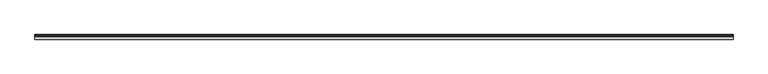
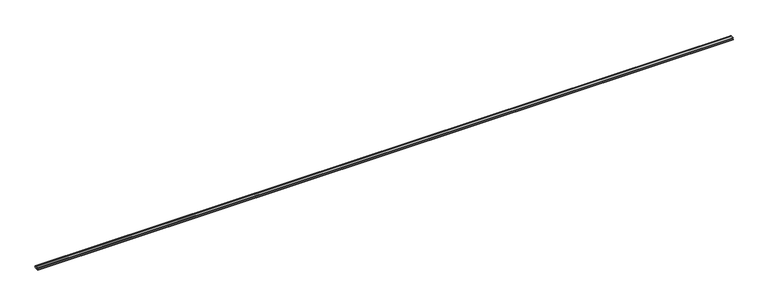
"""IFC4 building model written with IfcOpenShell, lengths in millimetres: proxy geometry, Generic Models 6:Generic Models 2:318829:Generic Models 2:318829 : Generic Models 6:Generic Models 2:318829:8 : Generic Models 6:Generic Models 2:318829:Generic Models 2:318829 : Generic Models 6:Generic Models 2:318829:300683."""

import ifcopenshell
import ifcopenshell.guid

model = None  # the IFC model being written
_history = None  # IfcOwnerHistory: only IFC2X3 demands one
_inside = {}  # id of a spatial element -> (the spatial element, [elements in it])
_under = {}  # id of a project, library or spatial element -> (it, [spatial elements below it])
_declared = {}  # id of a project -> (the project, [libraries it declares])
_typed = {}  # id of a type object -> (the type object, [elements of that type])
_made_of = {}  # id of a material, layer set ... -> (it, [elements and type objects made of it])


def new_model(schema):
    """Start an empty IFC model of exactly this schema.

    Asked for "IFC4X3", IfcOpenShell would pick the latest addendum, in which some entities
    have other attributes; the version numbers below select the first issue.
    IFC2X3 requires an IfcOwnerHistory on every rooted entity: one is made here for all.
    """
    global model, _history
    if schema == "IFC4X3":
        model = ifcopenshell.file(schema_version=(4, 3, 0, 0))
    else:
        model = ifcopenshell.file(schema=schema)
    _inside.clear()
    _under.clear()
    _declared.clear()
    _typed.clear()
    _made_of.clear()
    _history = None
    if model.schema == "IFC2X3":
        org = make("IfcOrganization", Name="unknown")
        user = make(
            "IfcPersonAndOrganization",
            ThePerson=make("IfcPerson", FamilyName="unknown"),
            TheOrganization=org,
        )
        app = make(
            "IfcApplication",
            ApplicationDeveloper=org,
            Version="unknown",
            ApplicationFullName="unknown",
            ApplicationIdentifier="unknown",
        )
        _history = make(
            "IfcOwnerHistory",
            OwningUser=user,
            OwningApplication=app,
            ChangeAction="ADDED",
            CreationDate=0,
        )
    return model


def make(cls, **values):
    """One entity of the class cls with the attributes given. An attribute that is None is left unset."""
    return model.create_entity(
        cls, **{name: value for name, value in values.items() if value is not None}
    )


def rooted(cls, **values):
    """An entity with a GlobalId (a new one), such as an element, a storey or a relation."""
    return make(cls, GlobalId=ifcopenshell.guid.new(), OwnerHistory=_history, **values)


def si_unit(unit_type, name, prefix=None):
    """IfcSIUnit, for example si_unit("LENGTHUNIT", "METRE", prefix="MILLI")."""
    return make("IfcSIUnit", UnitType=unit_type, Prefix=prefix, Name=name)


def assignment(units):
    """IfcUnitAssignment: the units of a project."""
    return None if units is None else make("IfcUnitAssignment", Units=units)


def point(xyz):
    """IfcCartesianPoint."""
    return None if xyz is None else make("IfcCartesianPoint", Coordinates=xyz)


def direction(xyz):
    """IfcDirection."""
    return None if xyz is None else make("IfcDirection", DirectionRatios=xyz)


def frame(location, z_axis=None, x_axis=None):
    """IfcAxis2Placement3D, a coordinate frame: its origin and axes. An axis left out is left unset."""
    return make(
        "IfcAxis2Placement3D",
        Location=point(location),
        Axis=direction(z_axis),
        RefDirection=direction(x_axis),
    )


def origin():
    """The frame at (0, 0, 0) with its axes left unset."""
    return frame((0.0, 0.0, 0.0))


def place(relative_to, where):
    """IfcLocalPlacement: puts the frame where relative to a parent placement (None: the world)."""
    return make(
        "IfcLocalPlacement", PlacementRelTo=relative_to, RelativePlacement=where
    )


def context(
    kind, dimensions, precision=None, world=None, true_north=None, identifier=None
):
    """IfcGeometricRepresentationContext, for example the 3D "Model" context."""
    return make(
        "IfcGeometricRepresentationContext",
        ContextIdentifier=identifier,
        ContextType=kind,
        CoordinateSpaceDimension=dimensions,
        Precision=precision,
        WorldCoordinateSystem=world,
        TrueNorth=true_north,
    )


def project(units=None, contexts=None):
    """IfcProject with its units and contexts."""
    return rooted(
        "IfcProject",
        Name="project",
        RepresentationContexts=contexts,
        UnitsInContext=assignment(units),
    )


def spatial(cls, under=None, at=None, **own):
    """A site, building, storey or space (cls), placed at a placement, below another one or the project."""
    s = rooted(cls, ObjectPlacement=at, **own)
    if under is not None:
        _under.setdefault(under.id(), (under, []))[1].append(s)
    return s


def polyline(points):
    """IfcPolyline through the points."""
    return make("IfcPolyline", Points=[point(p) for p in points])


def outline(outer, holes=None, kind="AREA"):
    """IfcArbitraryClosedProfileDef: a profile drawn as a closed curve; with holes, ...WithVoids."""
    if holes is None:
        return make("IfcArbitraryClosedProfileDef", ProfileType=kind, OuterCurve=outer)
    return make(
        "IfcArbitraryProfileDefWithVoids",
        ProfileType=kind,
        OuterCurve=outer,
        InnerCurves=holes,
    )


def extrude(swept, where, along, depth):
    """IfcExtrudedAreaSolid: the profile swept, set in the frame where, extruded along a direction by depth."""
    return make(
        "IfcExtrudedAreaSolid",
        SweptArea=swept,
        Position=where,
        ExtrudedDirection=direction(along),
        Depth=depth,
    )


def shape(context_of_items, identifier, shape_type, items):
    """IfcShapeRepresentation: the items that make up one representation, for example the "Body"."""
    return make(
        "IfcShapeRepresentation",
        ContextOfItems=context_of_items,
        RepresentationIdentifier=identifier,
        RepresentationType=shape_type,
        Items=items,
    )


def source(mapping_origin, context_of_items, identifier, shape_type, items):
    """IfcRepresentationMap: a shape defined once, which mapped items show again and again."""
    return make(
        "IfcRepresentationMap",
        MappingOrigin=mapping_origin,
        MappedRepresentation=shape(context_of_items, identifier, shape_type, items),
    )


def transform(
    local_origin,
    x_axis=None,
    y_axis=None,
    z_axis=None,
    scale=None,
    scale2=None,
    scale3=None,
    uniform=True,
):
    """IfcCartesianTransformationOperator3D, or its non-uniform kind. x_axis, y_axis, z_axis: its Axis1, 2, 3."""
    if uniform:
        return make(
            "IfcCartesianTransformationOperator3D",
            Axis1=direction(x_axis),
            Axis2=direction(y_axis),
            LocalOrigin=point(local_origin),
            Scale=scale,
            Axis3=direction(z_axis),
        )
    return make(
        "IfcCartesianTransformationOperator3DnonUniform",
        Axis1=direction(x_axis),
        Axis2=direction(y_axis),
        LocalOrigin=point(local_origin),
        Scale=scale,
        Axis3=direction(z_axis),
        Scale2=scale2,
        Scale3=scale3,
    )


def mapped(mapping_source, mapping_target):
    """IfcMappedItem: shows the shape of a source again, moved by a transform."""
    return make(
        "IfcMappedItem", MappingSource=mapping_source, MappingTarget=mapping_target
    )


def made_of(thing, what):
    """Note that an element or type object is made of a material, layer set ...; save() writes the relation."""
    if what is not None:
        _made_of.setdefault(what.id(), (what, []))[1].append(thing)
    return thing


def element(
    cls,
    number,
    at=None,
    inside=None,
    cuts=None,
    type_object=None,
    material=None,
    context=None,
    identifier="Body",
    shape_type=None,
    held_by="IfcProductDefinitionShape",
    body=None,
    shapes=None,
    **own,
):
    """One element of the class cls, such as IfcWall. Its Tag is "e" and its number.

    at: its placement. inside: the storey or other place that contains it. cuts: it is an
    opening in that element (IfcRelVoidsElement). A single representation is given by context,
    identifier, shape_type and body (its items); several are given by shapes. held_by: the class
    of the entity that holds the representations. save() writes the other relations.
    """
    e = rooted(cls, Tag="e%d" % number, ObjectPlacement=at, **own)
    if body is not None:
        shapes = [shape(context, identifier, shape_type, body)]
    if shapes is not None:
        e.Representation = make(held_by, Representations=shapes)
    if inside is not None:
        _inside.setdefault(inside.id(), (inside, []))[1].append(e)
    if cuts is not None:
        rooted(
            "IfcRelVoidsElement", RelatingBuildingElement=cuts, RelatedOpeningElement=e
        )
    if type_object is not None:
        _typed.setdefault(type_object.id(), (type_object, []))[1].append(e)
    return made_of(e, material)


def aggregate(whole, parts):
    """IfcRelAggregates: a whole, such as a stair, and the parts it consists of."""
    return rooted("IfcRelAggregates", RelatingObject=whole, RelatedObjects=parts)


def save(model, path):
    """Write the relations noted so far, then the file.

    IfcRelAggregates (storeys below a building ...), IfcRelContainedInSpatialStructure (elements
    in a storey), IfcRelDefinesByType, IfcRelAssociatesMaterial and IfcRelDeclares: one each for
    every whole, place, type object, material and project.
    """
    for whole, parts in _under.values():
        aggregate(whole, parts)
    for where, things in _inside.values():
        rooted(
            "IfcRelContainedInSpatialStructure",
            RelatedElements=things,
            RelatingStructure=where,
        )
    for kind, things in _typed.values():
        rooted("IfcRelDefinesByType", RelatedObjects=things, RelatingType=kind)
    for what, things in _made_of.values():
        rooted("IfcRelAssociatesMaterial", RelatedObjects=things, RelatingMaterial=what)
    for by, libraries in _declared.values():
        rooted("IfcRelDeclares", RelatingContext=by, RelatedDefinitions=libraries)
    model.write(path)


def generic_models_16859b6c(model_context):
    return source(origin(), model_context, "Body", "SweptSolid", [
        extrude(outline(polyline([(-579078.7997973, 0.0), (-579086.1349125, 0.0), (-579085.6631517, 1.207204), (-579085.2710441, 3.96875), (-579085.6631517, 6.730296), (-579086.1349125, 7.9375), (-579078.7997973, 7.9375), (-579080.7913182, 6.834014), (-579082.0090745, 5.2822838), (-579082.2625594, 3.5250635), (-579081.5121175, 1.8372538), (-579079.8751485, 0.482897), (-579078.7997973, 0.0)])), frame((590317.0242239, 0.0, 0.0), z_axis=(1.0, 0.0, 0.0), x_axis=(0.0, 1.0, 0.0)), (0.0, 0.0, 1.0), 2438.4),
        extrude(outline(polyline([(-579074.5205679, 0.0995049), (-579075.8452628, 0.0), (-579077.1699578, 0.0995049), (-579079.5569756, 0.8658563), (-579081.2088431, 2.2467739), (-579081.7983878, 3.96875), (-579081.2088431, 5.6907261), (-579079.5569756, 7.0716437), (-579077.1699578, 7.8379952), (-579075.8452628, 7.9375), (-579074.5205679, 7.8379952), (-579072.1335501, 7.0716437), (-579070.4816826, 5.6907261), (-579069.8921378, 3.96875), (-579070.4816826, 2.2467739), (-579072.1335501, 0.8658563), (-579074.5205679, 0.0995049)])), frame((590317.0242239, 0.0, 0.0), z_axis=(1.0, 0.0, 0.0), x_axis=(0.0, 1.0, 0.0)), (0.0, 0.0, 1.0), 2438.4),
    ])


if __name__ == "__main__":
    model = new_model("IFC4")
    model_context = context("Model", 3, world=origin())
    ifc_project = project(units=[si_unit("LENGTHUNIT", "METRE", prefix="MILLI")], contexts=[model_context])
    site = spatial("IfcSite", under=ifc_project)
    building = spatial("IfcBuilding", under=site)
    placement = place(None, origin())
    generic_models_shape = generic_models_16859b6c(model_context)
    element("IfcBuildingElementProxy", 1, Name="Generic Models 6:Generic Models 2:318829:Generic Models 2:318829 : Generic Models 6:Generic Models 2:318829:8 : Generic Models 6:Generic Models 2:318829:Generic Models 2:318829 : Generic Models 6:Generic Models 2:318829:300683", ObjectType="Generic Models 6:Generic Models 2:318829:Generic Models 2:318829 : Generic Models 6:Generic Models 2:318829:8 : Generic Models 6:Generic Models 2:318829:Generic Models 2:318829 : Generic Models 6:Generic Models 2:318829:300683", at=placement, inside=building, context=model_context, shape_type="MappedRepresentation", body=[
        mapped(generic_models_shape, transform((0.0, 0.0, 0.0), x_axis=(1.0, 0.0, 0.0), y_axis=(0.0, 1.0, 0.0), z_axis=(0.0, 0.0, 1.0))),
    ])
    save(model, "model.ifc")

# Revit data of these elements
# Type "Generic Models 6:Generic Models 2:318829:Generic Models 2:318829 : Generic Models 6:Generic Models 2:318829:8 : Generic Models 6:Generic Models 2:318829:Generic Models 2:318829 : Generic Models 6:Generic Models 2:318829:300683"
#   NameOverride = "Generic Models 6:Generic Models 2:318829:Generic Models 2:318829 : Generic Models 6:Generic Models 2:318829:300683"
#   ObjectTypeOverride = "Generic Models 2:318829 : Generic Models 6:Generic Models 2:318829"
#   Reference = "Generic Models 2"
#   Tag = "300683"
# Element 1 (IfcBuildingElementProxy, "Generic Models 6:Generic Models 2:318829:Generic Models 2:318829 : Generic Models 6:Generic Models 2:318829:8 : Generic Models 6:Generic Models 2:318829:Generic Models 2:318829 : Generic Models 6:Generic Models 2:318829:300683")
#   Materials on its faces: "SEALANT & BACKER ROD"
# Materials
#   "SEALANT & BACKER ROD": class "Unassigned", colour RGB 120 120 120, transparency 0, Cost = 0
